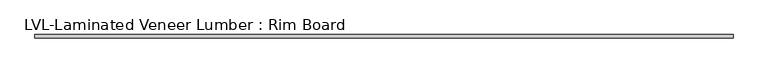
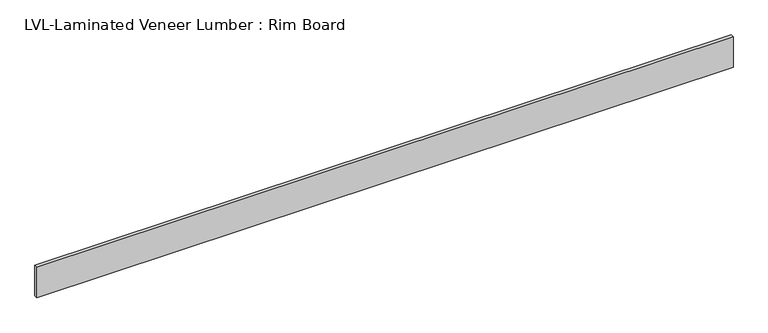
"""IFC4 building model written with IfcOpenShell, lengths in millimetres: beam geometry, LVL-Laminated Veneer Lumber : Rim Board."""

import ifcopenshell
import ifcopenshell.guid

model = None  # the IFC model being written
_history = None  # IfcOwnerHistory: only IFC2X3 demands one
_inside = {}  # id of a spatial element -> (the spatial element, [elements in it])
_under = {}  # id of a project, library or spatial element -> (it, [spatial elements below it])
_declared = {}  # id of a project -> (the project, [libraries it declares])
_typed = {}  # id of a type object -> (the type object, [elements of that type])
_made_of = {}  # id of a material, layer set ... -> (it, [elements and type objects made of it])


def new_model(schema):
    """Start an empty IFC model of exactly this schema.

    Asked for "IFC4X3", IfcOpenShell would pick the latest addendum, in which some entities
    have other attributes; the version numbers below select the first issue.
    IFC2X3 requires an IfcOwnerHistory on every rooted entity: one is made here for all.
    """
    global model, _history
    if schema == "IFC4X3":
        model = ifcopenshell.file(schema_version=(4, 3, 0, 0))
    else:
        model = ifcopenshell.file(schema=schema)
    _inside.clear()
    _under.clear()
    _declared.clear()
    _typed.clear()
    _made_of.clear()
    _history = None
    if model.schema == "IFC2X3":
        org = make("IfcOrganization", Name="unknown")
        user = make(
            "IfcPersonAndOrganization",
            ThePerson=make("IfcPerson", FamilyName="unknown"),
            TheOrganization=org,
        )
        app = make(
            "IfcApplication",
            ApplicationDeveloper=org,
            Version="unknown",
            ApplicationFullName="unknown",
            ApplicationIdentifier="unknown",
        )
        _history = make(
            "IfcOwnerHistory",
            OwningUser=user,
            OwningApplication=app,
            ChangeAction="ADDED",
            CreationDate=0,
        )
    return model


def make(cls, **values):
    """One entity of the class cls with the attributes given. An attribute that is None is left unset."""
    return model.create_entity(
        cls, **{name: value for name, value in values.items() if value is not None}
    )


def rooted(cls, **values):
    """An entity with a GlobalId (a new one), such as an element, a storey or a relation."""
    return make(cls, GlobalId=ifcopenshell.guid.new(), OwnerHistory=_history, **values)


def si_unit(unit_type, name, prefix=None):
    """IfcSIUnit, for example si_unit("LENGTHUNIT", "METRE", prefix="MILLI")."""
    return make("IfcSIUnit", UnitType=unit_type, Prefix=prefix, Name=name)


def assignment(units):
    """IfcUnitAssignment: the units of a project."""
    return None if units is None else make("IfcUnitAssignment", Units=units)


def point(xyz):
    """IfcCartesianPoint."""
    return None if xyz is None else make("IfcCartesianPoint", Coordinates=xyz)


def direction(xyz):
    """IfcDirection."""
    return None if xyz is None else make("IfcDirection", DirectionRatios=xyz)


def frame(location, z_axis=None, x_axis=None):
    """IfcAxis2Placement3D, a coordinate frame: its origin and axes. An axis left out is left unset."""
    return make(
        "IfcAxis2Placement3D",
        Location=point(location),
        Axis=direction(z_axis),
        RefDirection=direction(x_axis),
    )


def origin():
    """The frame at (0, 0, 0) with its axes left unset."""
    return frame((0.0, 0.0, 0.0))


def place(relative_to, where):
    """IfcLocalPlacement: puts the frame where relative to a parent placement (None: the world)."""
    return make(
        "IfcLocalPlacement", PlacementRelTo=relative_to, RelativePlacement=where
    )


def context(
    kind, dimensions, precision=None, world=None, true_north=None, identifier=None
):
    """IfcGeometricRepresentationContext, for example the 3D "Model" context."""
    return make(
        "IfcGeometricRepresentationContext",
        ContextIdentifier=identifier,
        ContextType=kind,
        CoordinateSpaceDimension=dimensions,
        Precision=precision,
        WorldCoordinateSystem=world,
        TrueNorth=true_north,
    )


def project(units=None, contexts=None):
    """IfcProject with its units and contexts."""
    return rooted(
        "IfcProject",
        Name="project",
        RepresentationContexts=contexts,
        UnitsInContext=assignment(units),
    )


def spatial(cls, under=None, at=None, **own):
    """A site, building, storey or space (cls), placed at a placement, below another one or the project."""
    s = rooted(cls, ObjectPlacement=at, **own)
    if under is not None:
        _under.setdefault(under.id(), (under, []))[1].append(s)
    return s


def polyline(points):
    """IfcPolyline through the points."""
    return make("IfcPolyline", Points=[point(p) for p in points])


def outline(outer, holes=None, kind="AREA"):
    """IfcArbitraryClosedProfileDef: a profile drawn as a closed curve; with holes, ...WithVoids."""
    if holes is None:
        return make("IfcArbitraryClosedProfileDef", ProfileType=kind, OuterCurve=outer)
    return make(
        "IfcArbitraryProfileDefWithVoids",
        ProfileType=kind,
        OuterCurve=outer,
        InnerCurves=holes,
    )


def extrude(swept, where, along, depth):
    """IfcExtrudedAreaSolid: the profile swept, set in the frame where, extruded along a direction by depth."""
    return make(
        "IfcExtrudedAreaSolid",
        SweptArea=swept,
        Position=where,
        ExtrudedDirection=direction(along),
        Depth=depth,
    )


def shape(context_of_items, identifier, shape_type, items):
    """IfcShapeRepresentation: the items that make up one representation, for example the "Body"."""
    return make(
        "IfcShapeRepresentation",
        ContextOfItems=context_of_items,
        RepresentationIdentifier=identifier,
        RepresentationType=shape_type,
        Items=items,
    )


def source(mapping_origin, context_of_items, identifier, shape_type, items):
    """IfcRepresentationMap: a shape defined once, which mapped items show again and again."""
    return make(
        "IfcRepresentationMap",
        MappingOrigin=mapping_origin,
        MappedRepresentation=shape(context_of_items, identifier, shape_type, items),
    )


def transform(
    local_origin,
    x_axis=None,
    y_axis=None,
    z_axis=None,
    scale=None,
    scale2=None,
    scale3=None,
    uniform=True,
):
    """IfcCartesianTransformationOperator3D, or its non-uniform kind. x_axis, y_axis, z_axis: its Axis1, 2, 3."""
    if uniform:
        return make(
            "IfcCartesianTransformationOperator3D",
            Axis1=direction(x_axis),
            Axis2=direction(y_axis),
            LocalOrigin=point(local_origin),
            Scale=scale,
            Axis3=direction(z_axis),
        )
    return make(
        "IfcCartesianTransformationOperator3DnonUniform",
        Axis1=direction(x_axis),
        Axis2=direction(y_axis),
        LocalOrigin=point(local_origin),
        Scale=scale,
        Axis3=direction(z_axis),
        Scale2=scale2,
        Scale3=scale3,
    )


def mapped(mapping_source, mapping_target):
    """IfcMappedItem: shows the shape of a source again, moved by a transform."""
    return make(
        "IfcMappedItem", MappingSource=mapping_source, MappingTarget=mapping_target
    )


def made_of(thing, what):
    """Note that an element or type object is made of a material, layer set ...; save() writes the relation."""
    if what is not None:
        _made_of.setdefault(what.id(), (what, []))[1].append(thing)
    return thing


def element(
    cls,
    number,
    at=None,
    inside=None,
    cuts=None,
    type_object=None,
    material=None,
    context=None,
    identifier="Body",
    shape_type=None,
    held_by="IfcProductDefinitionShape",
    body=None,
    shapes=None,
    **own,
):
    """One element of the class cls, such as IfcWall. Its Tag is "e" and its number.

    at: its placement. inside: the storey or other place that contains it. cuts: it is an
    opening in that element (IfcRelVoidsElement). A single representation is given by context,
    identifier, shape_type and body (its items); several are given by shapes. held_by: the class
    of the entity that holds the representations. save() writes the other relations.
    """
    e = rooted(cls, Tag="e%d" % number, ObjectPlacement=at, **own)
    if body is not None:
        shapes = [shape(context, identifier, shape_type, body)]
    if shapes is not None:
        e.Representation = make(held_by, Representations=shapes)
    if inside is not None:
        _inside.setdefault(inside.id(), (inside, []))[1].append(e)
    if cuts is not None:
        rooted(
            "IfcRelVoidsElement", RelatingBuildingElement=cuts, RelatedOpeningElement=e
        )
    if type_object is not None:
        _typed.setdefault(type_object.id(), (type_object, []))[1].append(e)
    return made_of(e, material)


def aggregate(whole, parts):
    """IfcRelAggregates: a whole, such as a stair, and the parts it consists of."""
    return rooted("IfcRelAggregates", RelatingObject=whole, RelatedObjects=parts)


def save(model, path):
    """Write the relations noted so far, then the file.

    IfcRelAggregates (storeys below a building ...), IfcRelContainedInSpatialStructure (elements
    in a storey), IfcRelDefinesByType, IfcRelAssociatesMaterial and IfcRelDeclares: one each for
    every whole, place, type object, material and project.
    """
    for whole, parts in _under.values():
        aggregate(whole, parts)
    for where, things in _inside.values():
        rooted(
            "IfcRelContainedInSpatialStructure",
            RelatedElements=things,
            RelatingStructure=where,
        )
    for kind, things in _typed.values():
        rooted("IfcRelDefinesByType", RelatedObjects=things, RelatingType=kind)
    for what, things in _made_of.values():
        rooted("IfcRelAssociatesMaterial", RelatedObjects=things, RelatingMaterial=what)
    for by, libraries in _declared.values():
        rooted("IfcRelDeclares", RelatingContext=by, RelatedDefinitions=libraries)
    model.write(path)


def lvl_laminated_veneer_lumber_rim_board_6caa49f5(model_context):
    return source(origin(), model_context, "Body", "SweptSolid", [
        extrude(outline(polyline([(3288.50625, 15.875), (3288.50625, -15.875), (-3288.50625, -15.875), (-3288.50625, 15.875), (3288.50625, 15.875)])), frame((0.0, 0.0, -150.8125), z_axis=(0.0, 0.0, 1.0), x_axis=(1.0, 0.0, 0.0)), (0.0, 0.0, 1.0), 301.625),
    ])


if __name__ == "__main__":
    model = new_model("IFC4")
    model_context = context("Model", 3, world=origin())
    ifc_project = project(units=[si_unit("LENGTHUNIT", "METRE", prefix="MILLI")], contexts=[model_context])
    site = spatial("IfcSite", under=ifc_project)
    building = spatial("IfcBuilding", under=site)
    placement = place(None, origin())
    lvl_laminated_veneer_lumber_rim_board_shape = lvl_laminated_veneer_lumber_rim_board_6caa49f5(model_context)
    element("IfcBeam", 1, ObjectType="LVL-Laminated Veneer Lumber : Rim Board", at=placement, inside=building, context=model_context, shape_type="MappedRepresentation", body=[
        mapped(lvl_laminated_veneer_lumber_rim_board_shape, transform((0.0, 0.0, 0.0), x_axis=(1.0, 0.0, 0.0), y_axis=(0.0, 1.0, 0.0), z_axis=(0.0, 0.0, 1.0))),
    ])
    save(model, "model.ifc")

# Revit data of these elements
# Type "LVL-Laminated Veneer Lumber : Rim Board"
#   Assembly Code = "B10"
#   Cost = 4.6
#   Length [instance default] = 5' - 0"
#   b = 0' - 1 1/4"
#   d = 0' - 11 7/8"
#   Structural Material [instance default] = Softwood, Lumber
# Element 1 (IfcBeam, "LVL-Laminated Veneer Lumber : Rim Board")
#   Structural Material = Douglas Fir #2
#   Materials on its faces: "Douglas Fir #2"
# Materials
#   "Softwood, Lumber": class "Wood", colour RGB 223 192 134, transparency 0, Description = "Pinus Echinata", Cost = 0
#   "Douglas Fir #2": class "Wood", colour RGB 223 192 134, transparency 0, Description = "Pinus Echinata", Cost = 0
